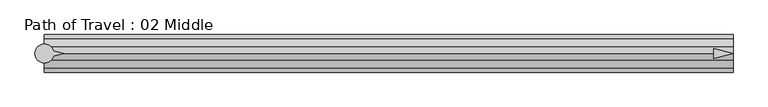
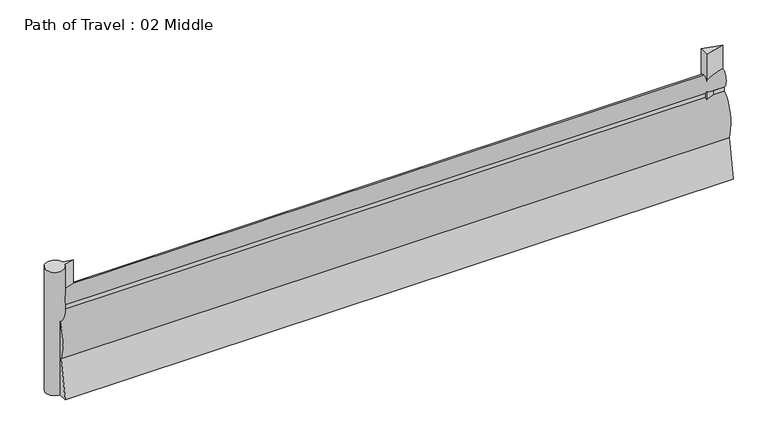
"""IFC4 building model written with IfcOpenShell, lengths in millimetres: proxy geometry, Path of Travel : 02 Middle."""

from ifc_helpers import new_model, si_unit, point, frame, frame_2d, origin, origin_with_axes, place, context, project, spatial, polyline, circle_curve, ellipse_curve, trimmed, segment, composite_curve, outline, extrude, source, transform, mapped, element, save
from ifc_brep_helpers import plane_surface, extruded_surface, advanced_brep


def path_of_travel_02_middle_ffbbecd6(model_context):
    return source(origin(), model_context, "Body", "SolidModel", [
        advanced_brep(
        [(227.5554837, 0.0, 1727.2), (227.5554837, 42.9018657, 1436.6534209), (227.5554837, 42.9018657, 1363.4763406), (227.5554837, 184.1186263, 643.4144547), (227.5554837, 297.5699544, 0.0), (227.5554837, 145.6574193, 0.0), (227.5554837, 0.0, 584.2), (227.5554837, -145.6574193, 0.0), (227.5554837, -297.5699544, 0.0), (227.5554837, -184.1186263, 643.4144547), (227.5554837, -42.9018657, 1363.4763406), (227.5554837, -42.9018657, 1436.6534209), (11129.056196, 0.0, 1727.2), (11129.056196, -42.9018657, 1436.6534209), (11129.056196, -42.9018657, 1363.4763406), (11129.056196, -184.1186263, 643.4144547), (11129.056196, -297.5699544, 0.0), (11129.056196, -145.6574193, 0.0), (11129.056196, 0.0, 584.2), (11129.056196, 145.6574193, 0.0), (11129.056196, 297.5699544, 0.0), (11129.056196, 184.1186263, 643.4144547), (11129.056196, 42.9018657, 1363.4763406), (11129.056196, 42.9018657, 1436.6534209)],
        [
            (0, 1, ellipse_curve(frame((227.5554837, 0.0, 1574.8), z_axis=(-1.0, 0.0, 0.0), x_axis=(0.0, 0.0, 1.0)), 152.4, 101.6)),
            (1, 2),
            (2, 3, ellipse_curve(frame((227.5554837, 0.0, 914.4), z_axis=(-1.0, 0.0, 0.0), x_axis=(0.0, 0.0, -1.0)), 457.2, 228.6)),
            (3, 4),
            (4, 5),
            (5, 6),
            (6, 7),
            (7, 8),
            (8, 9),
            (9, 10, ellipse_curve(frame((227.5554837, 0.0, 914.4), z_axis=(-1.0, 0.0, 0.0), x_axis=(0.0, 0.0, -1.0)), 457.2, 228.6)),
            (10, 11),
            (11, 0, ellipse_curve(frame((227.5554837, 0.0, 1574.8), z_axis=(-1.0, 0.0, 0.0), x_axis=(0.0, 0.0, 1.0)), 152.4, 101.6)),
            (12, 13, ellipse_curve(frame((11129.056196, 0.0, 1574.8), z_axis=(1.0, 0.0, 0.0), x_axis=(0.0, 0.0, 1.0)), 152.4, 101.6)),
            (13, 14),
            (14, 15, ellipse_curve(frame((11129.056196, 0.0, 914.4), z_axis=(1.0, 0.0, 0.0), x_axis=(0.0, 0.0, -1.0)), 457.2, 228.6)),
            (15, 16),
            (16, 17),
            (17, 18),
            (18, 19),
            (19, 20),
            (20, 21),
            (21, 22, ellipse_curve(frame((11129.056196, 0.0, 914.4), z_axis=(1.0, 0.0, 0.0), x_axis=(0.0, 0.0, -1.0)), 457.2, 228.6)),
            (22, 23),
            (23, 12, ellipse_curve(frame((11129.056196, 0.0, 1574.8), z_axis=(1.0, 0.0, 0.0), x_axis=(0.0, 0.0, 1.0)), 152.4, 101.6)),
            (0, 12),
            (23, 1),
            (22, 2),
            (21, 3),
            (20, 4),
            (19, 5),
            (18, 6),
            (17, 7),
            (16, 8),
            (15, 9),
            (14, 10),
            (13, 11),
        ],
        [
            plane_surface(frame((227.5554837, 0.0, 0.0), z_axis=(-1.0, 0.0, 0.0), x_axis=(0.0, 0.0, 1.0))),
            plane_surface(frame((11129.056196, 0.0, 0.0), z_axis=(1.0, 0.0, 0.0), x_axis=(0.0, 0.0, 1.0))),
            extruded_surface(trimmed(ellipse_curve(frame((11129.056196, 0.0, 1574.8), z_axis=(-1.0, 0.0, 0.0), x_axis=(0.0, 0.0, 1.0)), 152.4, 101.6), [point((11129.056196, 0.0, 1727.2))], [point((11129.056196, 42.9018657, 1436.6534209))], True, "CARTESIAN"), (-10901.5007123, 0.0, 0.0), 10901.5007123),
            plane_surface(frame((227.5554837, 42.9018657, 1436.6534209), z_axis=(0.0, 1.0, 0.0), x_axis=(1.0, 0.0, 0.0))),
            extruded_surface(trimmed(ellipse_curve(frame((11129.056196, 0.0, 914.4), z_axis=(-1.0, 0.0, 0.0), x_axis=(0.0, 0.0, -1.0)), 457.2, 228.6), [point((11129.056196, 42.9018657, 1363.4763406))], [point((11129.056196, 184.1186263, 643.4144547))], True, "CARTESIAN"), (-10901.5007123, 0.0, 0.0), 10901.5007123),
            plane_surface(frame((227.5554837, 184.1186263, 643.4144547), z_axis=(0.0, 0.9848077530122078, 0.1736481776669322), x_axis=(1.0, 0.0, 0.0))),
            plane_surface(frame((227.5554837, 297.5699544, 0.0), z_axis=(0.0, 0.0, -1.0), x_axis=(1.0, 0.0, 0.0))),
            plane_surface(frame((227.5554837, 145.6574193, 0.0), z_axis=(0.0, -0.9702957262760199, -0.2419218955995739), x_axis=(1.0, 0.0, 0.0))),
            plane_surface(frame((227.5554837, 0.0, 584.2), z_axis=(0.0, 0.9702957262759961, -0.24192189559966923), x_axis=(1.0, 0.0, 0.0))),
            plane_surface(frame((227.5554837, -145.6574193, 0.0), z_axis=(0.0, 0.0, -1.0), x_axis=(1.0, 0.0, 0.0))),
            plane_surface(frame((227.5554837, -297.5699544, 0.0), z_axis=(0.0, -0.984807753012208, 0.17364817766693066), x_axis=(1.0, 0.0, 0.0))),
            extruded_surface(trimmed(ellipse_curve(frame((11129.056196, 0.0, 914.4), z_axis=(-1.0, 0.0, 0.0), x_axis=(0.0, 0.0, -1.0)), 457.2, 228.6), [point((11129.056196, -184.1186263, 643.4144547))], [point((11129.056196, -42.9018657, 1363.4763406))], True, "CARTESIAN"), (-10901.5007123, 0.0, 0.0), 10901.5007123),
            plane_surface(frame((227.5554837, -42.9018657, 1363.4763406), z_axis=(0.0, -1.0, 0.0), x_axis=(1.0, 0.0, 0.0))),
            extruded_surface(trimmed(ellipse_curve(frame((11129.056196, 0.0, 1574.8), z_axis=(-1.0, 0.0, 0.0), x_axis=(0.0, 0.0, 1.0)), 152.4, 101.6), [point((11129.056196, -42.9018657, 1436.6534209))], [point((11129.056196, 0.0, 1727.2))], True, "CARTESIAN"), (-10901.5007123, 0.0, 0.0), 10901.5007123),
        ],
        [
            (0, [[1, 2, 3, 4, 5, 6, 7, 8, 9, 10, 11, 12]]),
            (1, [[13, 14, 15, 16, 17, 18, 19, 20, 21, 22, 23, 24]]),
            (2, [[-1, 25, -24, 26]]),
            (3, [[-2, -26, -23, 27]]),
            (4, [[-3, -27, -22, 28]]),
            (5, [[-4, -28, -21, 29]]),
            (6, [[-5, -29, -20, 30]]),
            (7, [[-6, -30, -19, 31]]),
            (8, [[-7, -31, -18, 32]]),
            (9, [[-8, -32, -17, 33]]),
            (10, [[-9, -33, -16, 34]]),
            (11, [[-10, -34, -15, 35]]),
            (12, [[-11, -35, -14, 36]]),
            (13, [[-12, -36, -13, -25]]),
        ],
    ),
        extrude(outline(polyline([(10823.0510494, 76.2006338), (11129.056196, 0.0), (10823.0510494, -76.2006338), (10823.0510494, 76.2006338)])), origin_with_axes(), (0.0, 0.0, 1.0), 2129.5973753),
        extrude(outline(composite_curve([segment(polyline([(372.7837828, 39.4440225), (531.182385, 0.0), (372.7837828, -39.4440225)]), True, "CONTINUOUS"), segment(trimmed(circle_curve(frame_2d((227.2200886, 0.0)), 150.8131956), [point((372.7837828, -39.4440225))], [point((372.7837828, 39.4440225))], False, "CARTESIAN"), True, "CONTINUOUS")], self_intersect=False)), origin_with_axes(), (0.0, 0.0, 1.0), 2129.5973753),
    ])


if __name__ == "__main__":
    model = new_model("IFC4")
    model_context = context("Model", 3, world=origin())
    ifc_project = project(units=[si_unit("LENGTHUNIT", "METRE", prefix="MILLI")], contexts=[model_context])
    site = spatial("IfcSite", under=ifc_project)
    building = spatial("IfcBuilding", under=site)
    placement = place(None, origin())
    path_of_travel_02_middle_shape = path_of_travel_02_middle_ffbbecd6(model_context)
    element("IfcBuildingElementProxy", 1, Name="Path of Travel : 02 Middle", ObjectType="Path of Travel : 02 Middle", at=placement, inside=building, context=model_context, shape_type="MappedRepresentation", body=[
        mapped(path_of_travel_02_middle_shape, transform((0.0, 0.0, 0.0), x_axis=(1.0, 0.0, 0.0), y_axis=(0.0, 1.0, 0.0), z_axis=(0.0, 0.0, 1.0))),
    ])
    save(model, "model.ifc")

# Revit data of these elements
# Type "Path of Travel : 02 Middle"
#   Path of Egress [instance default] = 4' - 0"
#   built-in parameter 1001306 [instance default] = 4 (stored number, unit not read)
#   Dot at Start = no
#   Arrow in Middle = yes
#   Arrow at End = no
#   Egress Path = none
# Element 1 (IfcBuildingElementProxy, "Path of Travel : 02 Middle")
#   Path of Egress = 35' - 9.19294"
#   built-in parameter 1001306 = 35.7661 (stored number, unit not read)
#   Materials on its faces: "Egress Path Solid", "solid"
# Materials
#   "Egress Path Solid": class "Unassigned", colour RGB 255 128 64, transparency 0.75, Comments = "Rendering appearance not upgraded "
#   "solid": class "Generic", colour RGB 120 120 120, transparency 0, Cost = 0
